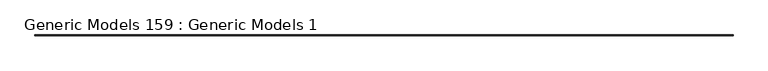
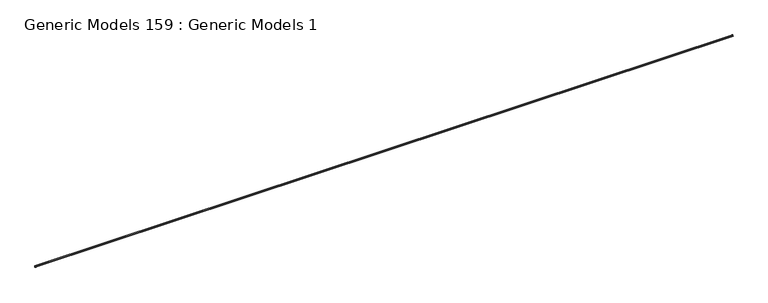
"""IFC4 building model written with IfcOpenShell, lengths in millimetres: proxy geometry, Generic Models 159 : Generic Models 1."""

from ifc_helpers import new_model, si_unit, frame, origin, place, context, project, spatial, polyline, outline, extrude, source, transform, mapped, element, save


def generic_models_159_generic_models_1_76a4f3de(model_context):
    return source(origin(), model_context, "Body", "SweptSolid", [
        extrude(outline(polyline([(6873.3019662, 124213.5950923), (6873.3019662, 124174.2250923), (6872.0319662, 124174.2250923), (6872.0319662, 124193.2750923), (6852.3469662, 124193.2750923), (6852.3469662, 124189.7952923), (6851.0769662, 124189.7952923), (6851.0769662, 124194.5450923), (6872.0319662, 124194.5450923), (6872.0319662, 124213.5950923), (6873.3019662, 124213.5950923)])), frame((-10437.7171316, 0.0, 0.0), z_axis=(1.0, 0.0, 0.0), x_axis=(0.0, 1.0, 0.0)), (0.0, 0.0, 1.0), 19050.0),
    ])


if __name__ == "__main__":
    model = new_model("IFC4")
    model_context = context("Model", 3, world=origin())
    ifc_project = project(units=[si_unit("LENGTHUNIT", "METRE", prefix="MILLI")], contexts=[model_context])
    site = spatial("IfcSite", under=ifc_project)
    building = spatial("IfcBuilding", under=site)
    placement = place(None, origin())
    generic_models_159_generic_models_1_shape = generic_models_159_generic_models_1_76a4f3de(model_context)
    element("IfcBuildingElementProxy", 1, Name="Generic Models 159 : Generic Models 1", ObjectType="Generic Models 159 : Generic Models 1", at=placement, inside=building, context=model_context, shape_type="MappedRepresentation", body=[
        mapped(generic_models_159_generic_models_1_shape, transform((0.0, 0.0, 0.0), x_axis=(1.0, 0.0, 0.0), y_axis=(0.0, 1.0, 0.0), z_axis=(0.0, 0.0, 1.0))),
    ])
    save(model, "model.ifc")

# Revit data of these elements
# Element 1 (IfcBuildingElementProxy, "Generic Models 159 : Generic Models 1")
#   Materials on its faces: "_ 16 GA. COPPER VENTED T REVEAL BEAD"
# Materials
#   "_ 16 GA. COPPER VENTED T REVEAL BEAD": class "Generic", colour RGB 253 192 103, transparency 0, Cost = 0
